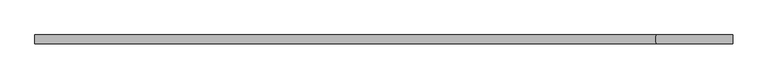
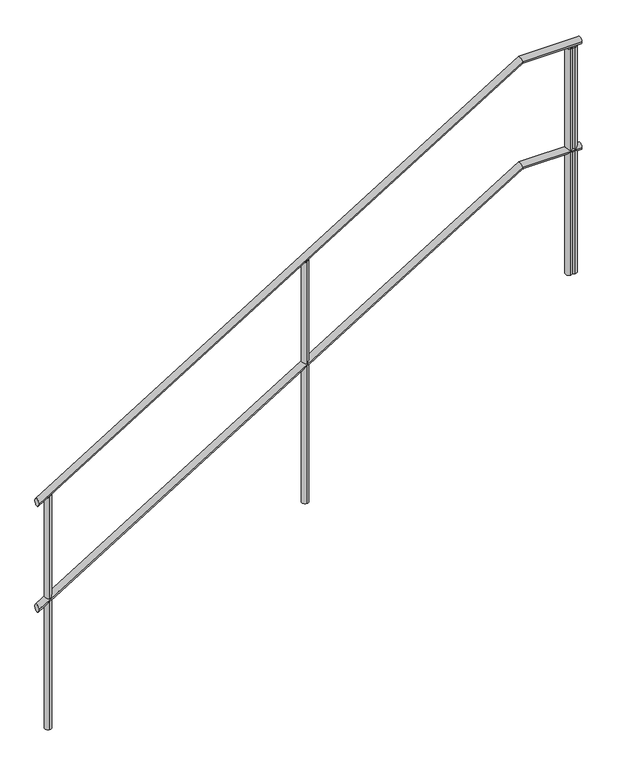
"""IFC4 building model written with IfcOpenShell, lengths in millimetres: railing geometry."""

from ifc_helpers import new_model, si_unit, point, frame, frame_2d, origin, place, context, project, spatial, circle_curve, ellipse_curve, trimmed, segment, composite_curve, outline, extrude, source, transform, mapped, element, save
from ifc_brep_helpers import plane_surface, cylinder_surface, advanced_brep


def railing_ba6ac100(model_context):
    return source(origin(), model_context, "Body", "SolidModel", [
        advanced_brep(
        [(3184.0, -687.9791411, -450.9609787), (3184.0, -717.9791411, -450.9609787), (5348.2567855, -717.9791411, 885.0), (5348.2567855, -687.9791411, 885.0), (5614.0, -687.9791411, 885.0), (5614.0, -717.9791411, 885.0)],
        [
            (0, 1, ellipse_curve(frame((3184.0, -702.9791411, -450.9609787), z_axis=(-1.0, 0.0, 0.0), x_axis=(0.0, 0.0, -1.0)), 17.6276454, 15.0)),
            (1, 0, ellipse_curve(frame((3184.0, -702.9791411, -450.9609787), z_axis=(-1.0, 0.0, 0.0), x_axis=(0.0, 0.0, -1.0)), 17.6276454, 15.0)),
            (1, 2),
            (2, 3, ellipse_curve(frame((5348.2567855, -702.9791411, 885.0), z_axis=(-0.9620125025549408, 0.0, -0.2730053935877092), x_axis=(0.2730053935877087, 0.0, -0.962012502554941)), 15.5923129, 15.0)),
            (3, 0),
            (3, 2, ellipse_curve(frame((5348.2567855, -702.9791411, 885.0), z_axis=(-0.9620125025549408, 0.0, -0.2730053935877092), x_axis=(0.2730053935877087, 0.0, -0.962012502554941)), 15.5923129, 15.0)),
            (4, 5, circle_curve(frame((5614.0, -702.9791411, 885.0), z_axis=(1.0, 0.0, 0.0), x_axis=(0.0, -1.0, 0.0)), 15.0)),
            (5, 4, circle_curve(frame((5614.0, -702.9791411, 885.0), z_axis=(1.0, 0.0, 0.0), x_axis=(0.0, -1.0, 0.0)), 15.0)),
            (2, 5),
            (4, 3),
        ],
        [
            plane_surface(frame((3184.0, -702.9791411, -433.3333333), z_axis=(-1.0, 0.0, 0.0), x_axis=(0.0, 1.0, 0.0))),
            cylinder_surface(frame((3191.8790381, -702.9791411, -446.097375), z_axis=(-0.8509361101440399, 0.0, -0.5252692037926174), x_axis=(0.0, -1.0, 0.0)), 15.0),
            plane_surface(frame((5614.0, -702.9791411, 900.0), z_axis=(1.0, 0.0, 0.0), x_axis=(0.0, 1.0, 0.0))),
            cylinder_surface(frame((5344.0, -702.9791411, 885.0), z_axis=(-1.0, 0.0, 0.0), x_axis=(0.0, -1.0, 0.0)), 15.0),
        ],
        [
            (0, [[1, 2]]),
            (1, [[-2, 3, 4, 5]]),
            (1, [[-1, -5, 6, -3]]),
            (2, [[7, 8]]),
            (3, [[-4, 9, -7, 10]]),
            (3, [[-6, -10, -8, -9]]),
        ],
    ),
        advanced_brep(
        [(3184.0, -687.9791411, 49.0390213), (3184.0, -717.9791411, 49.0390213), (5348.2567855, -717.9791411, 1385.0), (5348.2567855, -687.9791411, 1385.0), (5614.0, -687.9791411, 1385.0), (5614.0, -717.9791411, 1385.0)],
        [
            (0, 1, ellipse_curve(frame((3184.0, -702.9791411, 49.0390213), z_axis=(-1.0, 0.0, 0.0), x_axis=(0.0, 0.0, -1.0)), 17.6276454, 15.0)),
            (1, 0, ellipse_curve(frame((3184.0, -702.9791411, 49.0390213), z_axis=(-1.0, 0.0, 0.0), x_axis=(0.0, 0.0, -1.0)), 17.6276454, 15.0)),
            (1, 2),
            (2, 3, ellipse_curve(frame((5348.2567855, -702.9791411, 1385.0), z_axis=(-0.9620125025549408, 0.0, -0.2730053935877092), x_axis=(0.2730053935877087, 0.0, -0.962012502554941)), 15.5923129, 15.0)),
            (3, 0),
            (3, 2, ellipse_curve(frame((5348.2567855, -702.9791411, 1385.0), z_axis=(-0.9620125025549408, 0.0, -0.2730053935877092), x_axis=(0.2730053935877087, 0.0, -0.962012502554941)), 15.5923129, 15.0)),
            (4, 5, circle_curve(frame((5614.0, -702.9791411, 1385.0), z_axis=(1.0, 0.0, 0.0), x_axis=(0.0, -1.0, 0.0)), 15.0)),
            (5, 4, circle_curve(frame((5614.0, -702.9791411, 1385.0), z_axis=(1.0, 0.0, 0.0), x_axis=(0.0, -1.0, 0.0)), 15.0)),
            (2, 5),
            (4, 3),
        ],
        [
            plane_surface(frame((3184.0, -702.9791411, 66.6666667), z_axis=(-1.0, 0.0, 0.0), x_axis=(0.0, 1.0, 0.0))),
            cylinder_surface(frame((3191.8790381, -702.9791411, 53.902625), z_axis=(-0.8509361101440399, 0.0, -0.5252692037926174), x_axis=(0.0, -1.0, 0.0)), 15.0),
            plane_surface(frame((5614.0, -702.9791411, 1400.0), z_axis=(1.0, 0.0, 0.0), x_axis=(0.0, 1.0, 0.0))),
            cylinder_surface(frame((5344.0, -702.9791411, 1385.0), z_axis=(-1.0, 0.0, 0.0), x_axis=(0.0, -1.0, 0.0)), 15.0),
        ],
        [
            (0, [[1, 2]]),
            (1, [[-2, 3, 4, 5]]),
            (1, [[-1, -5, 6, -3]]),
            (2, [[7, 8]]),
            (3, [[-4, 9, -7, 10]]),
            (3, [[-6, -10, -8, -9]]),
        ],
    ),
        extrude(outline(composite_curve([segment(trimmed(circle_curve(frame_2d((5584.0, -702.9791411)), 15.0), [point((5584.0, -687.9791411))], [point((5584.0, -717.9791411))], False, "CARTESIAN"), True, "CONTINUOUS"), segment(trimmed(circle_curve(frame_2d((5584.0, -702.9791411)), 15.0), [point((5584.0, -717.9791411))], [point((5584.0, -687.9791411))], False, "CARTESIAN"), True, "CONTINUOUS")], self_intersect=False)), frame((0.0, 0.0, 300.0), z_axis=(0.0, 0.0, 1.0), x_axis=(1.0, 0.0, 0.0)), (0.0, 0.0, 1.0), 1070.0),
        advanced_brep(
        [(4384.0, -717.9791411, 777.4074074), (4384.0, -717.9791411, -366.6666667), (4384.0, -687.9791411, -366.6666667), (4384.0, -687.9791411, 777.4074074)],
        [
            (0, 1),
            (1, 2, circle_curve(frame((4384.0, -702.9791411, -366.6666667), z_axis=(0.0, 0.0, 1.0), x_axis=(0.0, 1.0, 0.0)), 15.0)),
            (2, 3),
            (3, 0, ellipse_curve(frame((4384.0, -702.9791411, 777.4074074), z_axis=(0.5252692037926167, 0.0, -0.8509361101440406), x_axis=(0.8509361101440406, 0.0, 0.5252692037926162)), 17.6276454, 15.0)),
            (0, 3, ellipse_curve(frame((4384.0, -702.9791411, 777.4074074), z_axis=(0.5252692037926167, 0.0, -0.8509361101440406), x_axis=(0.8509361101440406, 0.0, 0.5252692037926162)), 17.6276454, 15.0)),
            (2, 1, circle_curve(frame((4384.0, -702.9791411, -366.6666667), z_axis=(0.0, 0.0, 1.0), x_axis=(0.0, 1.0, 0.0)), 15.0)),
        ],
        [
            cylinder_surface(frame((4384.0, -702.9791411, -466.6666667), z_axis=(0.0, 0.0, 1.0), x_axis=(0.0, 1.0, 0.0)), 15.0),
            plane_surface(frame((4409.0, -677.9791411, 792.8395062), z_axis=(-0.5252692037926167, 0.0, 0.8509361101440406), x_axis=(0.0, -1.0, 0.0))),
            plane_surface(frame((4359.0, -677.9791411, -366.6666667), z_axis=(0.0, 0.0, -1.0), x_axis=(0.0, -1.0, 0.0))),
        ],
        [
            (0, [[1, 2, 3, 4]]),
            (0, [[-1, 5, -3, 6]]),
            (1, [[-4, -5]]),
            (2, [[-2, -6]]),
        ],
    ),
        extrude(outline(composite_curve([segment(trimmed(circle_curve(frame_2d((5564.0, -702.9791411)), 15.0), [point((5564.0, -687.9791411))], [point((5564.0, -717.9791411))], False, "CARTESIAN"), True, "CONTINUOUS"), segment(trimmed(circle_curve(frame_2d((5564.0, -702.9791411)), 15.0), [point((5564.0, -717.9791411))], [point((5564.0, -687.9791411))], False, "CARTESIAN"), True, "CONTINUOUS")], self_intersect=False)), frame((0.0, 0.0, 300.0), z_axis=(0.0, 0.0, 1.0), x_axis=(1.0, 0.0, 0.0)), (0.0, 0.0, 1.0), 1070.0),
        advanced_brep(
        [(3234.0, -717.9791411, 67.5308642), (3234.0, -717.9791411, -1033.3333333), (3234.0, -687.9791411, -1033.3333333), (3234.0, -687.9791411, 67.5308642)],
        [
            (0, 1),
            (1, 2, circle_curve(frame((3234.0, -702.9791411, -1033.3333333), z_axis=(0.0, 0.0, 1.0), x_axis=(0.0, 1.0, 0.0)), 15.0)),
            (2, 3),
            (3, 0, ellipse_curve(frame((3234.0, -702.9791411, 67.5308642), z_axis=(0.5252692037926167, 0.0, -0.8509361101440406), x_axis=(0.8509361101440406, 0.0, 0.5252692037926162)), 17.6276454, 15.0)),
            (0, 3, ellipse_curve(frame((3234.0, -702.9791411, 67.5308642), z_axis=(0.5252692037926167, 0.0, -0.8509361101440406), x_axis=(0.8509361101440406, 0.0, 0.5252692037926162)), 17.6276454, 15.0)),
            (2, 1, circle_curve(frame((3234.0, -702.9791411, -1033.3333333), z_axis=(0.0, 0.0, 1.0), x_axis=(0.0, 1.0, 0.0)), 15.0)),
        ],
        [
            cylinder_surface(frame((3234.0, -702.9791411, -1133.3333333), z_axis=(0.0, 0.0, 1.0), x_axis=(0.0, 1.0, 0.0)), 15.0),
            plane_surface(frame((3259.0, -677.9791411, 82.962963), z_axis=(-0.5252692037926167, 0.0, 0.8509361101440406), x_axis=(0.0, -1.0, 0.0))),
            plane_surface(frame((3209.0, -677.9791411, -1033.3333333), z_axis=(0.0, 0.0, -1.0), x_axis=(0.0, -1.0, 0.0))),
        ],
        [
            (0, [[1, 2, 3, 4]]),
            (0, [[-1, 5, -3, 6]]),
            (1, [[-4, -5]]),
            (2, [[-2, -6]]),
        ],
    ),
    ])


if __name__ == "__main__":
    model = new_model("IFC4")
    model_context = context("Model", 3, world=origin())
    ifc_project = project(units=[si_unit("LENGTHUNIT", "METRE", prefix="MILLI")], contexts=[model_context])
    site = spatial("IfcSite", under=ifc_project)
    building = spatial("IfcBuilding", under=site)
    placement = place(None, origin())
    railing_shape = railing_ba6ac100(model_context)
    element("IfcRailing", 1, at=placement, inside=building, context=model_context, shape_type="MappedRepresentation", body=[
        mapped(railing_shape, transform((0.0, 0.0, 0.0), x_axis=(1.0, 0.0, 0.0), y_axis=(0.0, 1.0, 0.0), z_axis=(0.0, 0.0, 1.0))),
    ])
    save(model, "model.ifc")
